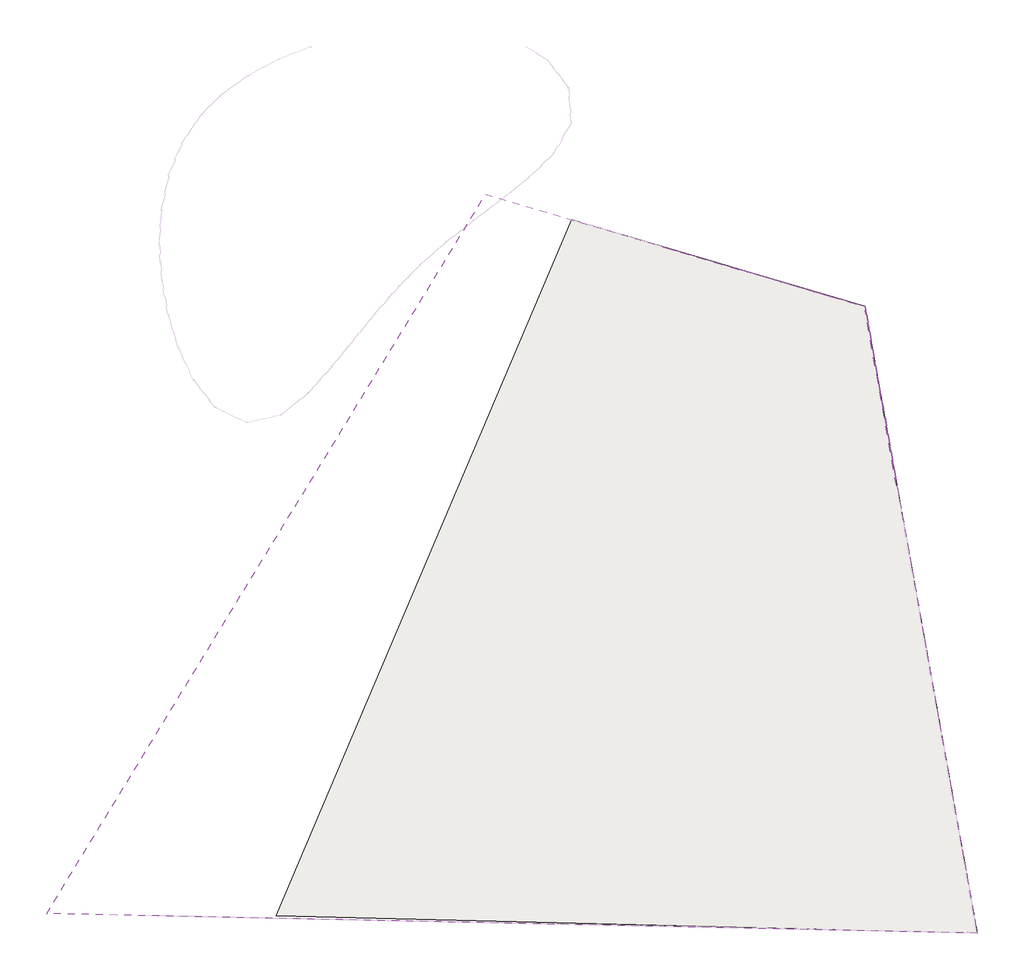
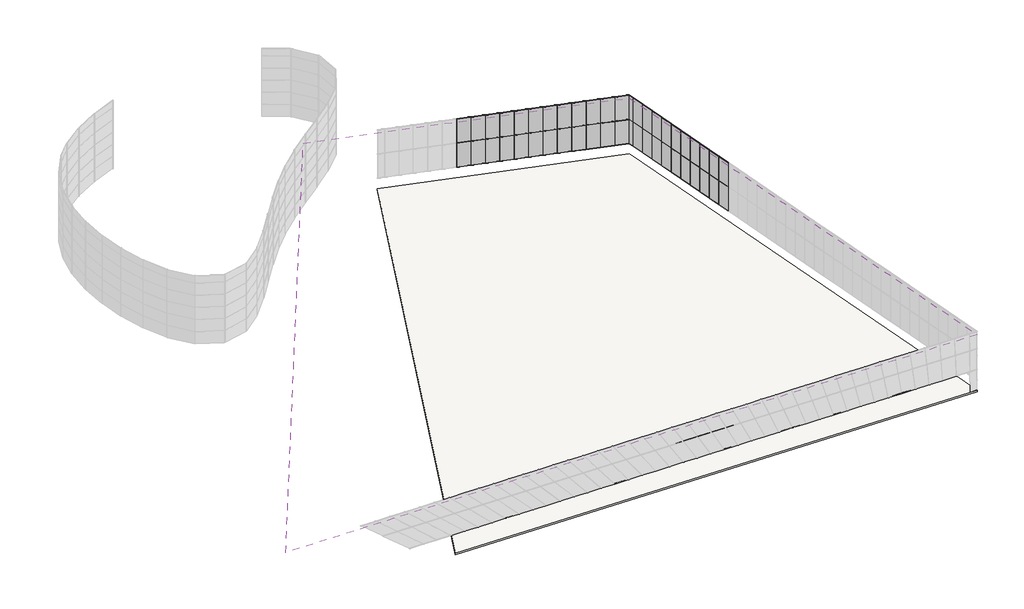
# One storey, part 8 of 8: 69 members, 46 plates, 1 roof, 1 slab.
"""IFC4 building model written with IfcOpenShell, lengths in millimetres."""

import ifcopenshell
import ifcopenshell.guid

model = None  # the IFC model being written
_history = None  # IfcOwnerHistory: only IFC2X3 demands one
_inside = {}  # id of a spatial element -> (the spatial element, [elements in it])
_under = {}  # id of a project, library or spatial element -> (it, [spatial elements below it])
_declared = {}  # id of a project -> (the project, [libraries it declares])
_typed = {}  # id of a type object -> (the type object, [elements of that type])
_made_of = {}  # id of a material, layer set ... -> (it, [elements and type objects made of it])


def new_model(schema):
    """Start an empty IFC model of exactly this schema.

    Asked for "IFC4X3", IfcOpenShell would pick the latest addendum, in which some entities
    have other attributes; the version numbers below select the first issue.
    IFC2X3 requires an IfcOwnerHistory on every rooted entity: one is made here for all.
    """
    global model, _history
    if schema == "IFC4X3":
        model = ifcopenshell.file(schema_version=(4, 3, 0, 0))
    else:
        model = ifcopenshell.file(schema=schema)
    _inside.clear()
    _under.clear()
    _declared.clear()
    _typed.clear()
    _made_of.clear()
    _history = None
    if model.schema == "IFC2X3":
        org = make("IfcOrganization", Name="unknown")
        user = make(
            "IfcPersonAndOrganization",
            ThePerson=make("IfcPerson", FamilyName="unknown"),
            TheOrganization=org,
        )
        app = make(
            "IfcApplication",
            ApplicationDeveloper=org,
            Version="unknown",
            ApplicationFullName="unknown",
            ApplicationIdentifier="unknown",
        )
        _history = make(
            "IfcOwnerHistory",
            OwningUser=user,
            OwningApplication=app,
            ChangeAction="ADDED",
            CreationDate=0,
        )
    return model


def make(cls, **values):
    """One entity of the class cls with the attributes given. An attribute that is None is left unset."""
    return model.create_entity(
        cls, **{name: value for name, value in values.items() if value is not None}
    )


def rooted(cls, **values):
    """An entity with a GlobalId (a new one), such as an element, a storey or a relation."""
    return make(cls, GlobalId=ifcopenshell.guid.new(), OwnerHistory=_history, **values)


def si_unit(unit_type, name, prefix=None):
    """IfcSIUnit, for example si_unit("LENGTHUNIT", "METRE", prefix="MILLI")."""
    return make("IfcSIUnit", UnitType=unit_type, Prefix=prefix, Name=name)


def assignment(units):
    """IfcUnitAssignment: the units of a project."""
    return None if units is None else make("IfcUnitAssignment", Units=units)


def point(xyz):
    """IfcCartesianPoint."""
    return None if xyz is None else make("IfcCartesianPoint", Coordinates=xyz)


def direction(xyz):
    """IfcDirection."""
    return None if xyz is None else make("IfcDirection", DirectionRatios=xyz)


def frame(location, z_axis=None, x_axis=None):
    """IfcAxis2Placement3D, a coordinate frame: its origin and axes. An axis left out is left unset."""
    return make(
        "IfcAxis2Placement3D",
        Location=point(location),
        Axis=direction(z_axis),
        RefDirection=direction(x_axis),
    )


def frame_2d(location, x_axis=None):
    """IfcAxis2Placement2D, a coordinate frame in the plane: its origin and x axis."""
    return make(
        "IfcAxis2Placement2D", Location=point(location), RefDirection=direction(x_axis)
    )


def origin():
    """The frame at (0, 0, 0) with its axes left unset."""
    return frame((0.0, 0.0, 0.0))


def origin_with_axes():
    """The frame at (0, 0, 0) with the z axis (0, 0, 1) and the x axis (1, 0, 0) written out."""
    return frame((0.0, 0.0, 0.0), z_axis=(0.0, 0.0, 1.0), x_axis=(1.0, 0.0, 0.0))


def origin_2d():
    """The frame at (0, 0) in the plane with its x axis left unset."""
    return frame_2d((0.0, 0.0))


def place(relative_to, where):
    """IfcLocalPlacement: puts the frame where relative to a parent placement (None: the world)."""
    return make(
        "IfcLocalPlacement", PlacementRelTo=relative_to, RelativePlacement=where
    )


def context(
    kind, dimensions, precision=None, world=None, true_north=None, identifier=None
):
    """IfcGeometricRepresentationContext, for example the 3D "Model" context."""
    return make(
        "IfcGeometricRepresentationContext",
        ContextIdentifier=identifier,
        ContextType=kind,
        CoordinateSpaceDimension=dimensions,
        Precision=precision,
        WorldCoordinateSystem=world,
        TrueNorth=true_north,
    )


def project(units=None, contexts=None):
    """IfcProject with its units and contexts."""
    return rooted(
        "IfcProject",
        Name="project",
        RepresentationContexts=contexts,
        UnitsInContext=assignment(units),
    )


def spatial(cls, under=None, at=None, **own):
    """A site, building, storey or space (cls), placed at a placement, below another one or the project."""
    s = rooted(cls, ObjectPlacement=at, **own)
    if under is not None:
        _under.setdefault(under.id(), (under, []))[1].append(s)
    return s


def polyline(points):
    """IfcPolyline through the points."""
    return make("IfcPolyline", Points=[point(p) for p in points])


def circle_curve(where, radius):
    """IfcCircle in the frame where."""
    return make("IfcCircle", Position=where, Radius=radius)


def trimmed(basis, trim1, trim2, sense, master):
    """IfcTrimmedCurve: the piece of a basis curve between two trims."""
    return make(
        "IfcTrimmedCurve",
        BasisCurve=basis,
        Trim1=trim1,
        Trim2=trim2,
        SenseAgreement=sense,
        MasterRepresentation=master,
    )


def segment(curve, same_sense, transition):
    """IfcCompositeCurveSegment."""
    return make(
        "IfcCompositeCurveSegment",
        Transition=transition,
        SameSense=same_sense,
        ParentCurve=curve,
    )


def composite_curve(segments, self_intersect=None):
    """IfcCompositeCurve: segments joined end to end."""
    return make("IfcCompositeCurve", Segments=segments, SelfIntersect=self_intersect)


def outline(outer, holes=None, kind="AREA"):
    """IfcArbitraryClosedProfileDef: a profile drawn as a closed curve; with holes, ...WithVoids."""
    if holes is None:
        return make("IfcArbitraryClosedProfileDef", ProfileType=kind, OuterCurve=outer)
    return make(
        "IfcArbitraryProfileDefWithVoids",
        ProfileType=kind,
        OuterCurve=outer,
        InnerCurves=holes,
    )


def extrude(swept, where, along, depth):
    """IfcExtrudedAreaSolid: the profile swept, set in the frame where, extruded along a direction by depth."""
    return make(
        "IfcExtrudedAreaSolid",
        SweptArea=swept,
        Position=where,
        ExtrudedDirection=direction(along),
        Depth=depth,
    )


def shape(context_of_items, identifier, shape_type, items):
    """IfcShapeRepresentation: the items that make up one representation, for example the "Body"."""
    return make(
        "IfcShapeRepresentation",
        ContextOfItems=context_of_items,
        RepresentationIdentifier=identifier,
        RepresentationType=shape_type,
        Items=items,
    )


def source(mapping_origin, context_of_items, identifier, shape_type, items):
    """IfcRepresentationMap: a shape defined once, which mapped items show again and again."""
    return make(
        "IfcRepresentationMap",
        MappingOrigin=mapping_origin,
        MappedRepresentation=shape(context_of_items, identifier, shape_type, items),
    )


def transform(
    local_origin,
    x_axis=None,
    y_axis=None,
    z_axis=None,
    scale=None,
    scale2=None,
    scale3=None,
    uniform=True,
):
    """IfcCartesianTransformationOperator3D, or its non-uniform kind. x_axis, y_axis, z_axis: its Axis1, 2, 3."""
    if uniform:
        return make(
            "IfcCartesianTransformationOperator3D",
            Axis1=direction(x_axis),
            Axis2=direction(y_axis),
            LocalOrigin=point(local_origin),
            Scale=scale,
            Axis3=direction(z_axis),
        )
    return make(
        "IfcCartesianTransformationOperator3DnonUniform",
        Axis1=direction(x_axis),
        Axis2=direction(y_axis),
        LocalOrigin=point(local_origin),
        Scale=scale,
        Axis3=direction(z_axis),
        Scale2=scale2,
        Scale3=scale3,
    )


def mapped(mapping_source, mapping_target):
    """IfcMappedItem: shows the shape of a source again, moved by a transform."""
    return make(
        "IfcMappedItem", MappingSource=mapping_source, MappingTarget=mapping_target
    )


def made_of(thing, what):
    """Note that an element or type object is made of a material, layer set ...; save() writes the relation."""
    if what is not None:
        _made_of.setdefault(what.id(), (what, []))[1].append(thing)
    return thing


def element(
    cls,
    number,
    at=None,
    inside=None,
    cuts=None,
    type_object=None,
    material=None,
    context=None,
    identifier="Body",
    shape_type=None,
    held_by="IfcProductDefinitionShape",
    body=None,
    shapes=None,
    **own,
):
    """One element of the class cls, such as IfcWall. Its Tag is "e" and its number.

    at: its placement. inside: the storey or other place that contains it. cuts: it is an
    opening in that element (IfcRelVoidsElement). A single representation is given by context,
    identifier, shape_type and body (its items); several are given by shapes. held_by: the class
    of the entity that holds the representations. save() writes the other relations.
    """
    e = rooted(cls, Tag="e%d" % number, ObjectPlacement=at, **own)
    if body is not None:
        shapes = [shape(context, identifier, shape_type, body)]
    if shapes is not None:
        e.Representation = make(held_by, Representations=shapes)
    if inside is not None:
        _inside.setdefault(inside.id(), (inside, []))[1].append(e)
    if cuts is not None:
        rooted(
            "IfcRelVoidsElement", RelatingBuildingElement=cuts, RelatedOpeningElement=e
        )
    if type_object is not None:
        _typed.setdefault(type_object.id(), (type_object, []))[1].append(e)
    return made_of(e, material)


def aggregate(whole, parts):
    """IfcRelAggregates: a whole, such as a stair, and the parts it consists of."""
    return rooted("IfcRelAggregates", RelatingObject=whole, RelatedObjects=parts)


def save(model, path):
    """Write the relations noted so far, then the file.

    IfcRelAggregates (storeys below a building ...), IfcRelContainedInSpatialStructure (elements
    in a storey), IfcRelDefinesByType, IfcRelAssociatesMaterial and IfcRelDeclares: one each for
    every whole, place, type object, material and project.
    """
    for whole, parts in _under.values():
        aggregate(whole, parts)
    for where, things in _inside.values():
        rooted(
            "IfcRelContainedInSpatialStructure",
            RelatedElements=things,
            RelatingStructure=where,
        )
    for kind, things in _typed.values():
        rooted("IfcRelDefinesByType", RelatedObjects=things, RelatingType=kind)
    for what, things in _made_of.values():
        rooted("IfcRelAssociatesMaterial", RelatedObjects=things, RelatingMaterial=what)
    for by, libraries in _declared.values():
        rooted("IfcRelDeclares", RelatingContext=by, RelatedDefinitions=libraries)
    model.write(path)


def montante_circular_25_mm_raio_666f7a7d(model_context):
    return source(origin(), model_context, "Body", "SweptSolid", [
        extrude(outline(composite_curve([segment(trimmed(circle_curve(frame_2d((-25.0, 0.0)), 25.0), [point((0.0, 0.0))], [point((-50.0, 0.0))], False, "CARTESIAN"), True, "CONTINUOUS"), segment(trimmed(circle_curve(frame_2d((-25.0, 0.0)), 25.0), [point((-50.0, 0.0))], [point((0.0, 0.0))], False, "CARTESIAN"), True, "CONTINUOUS")], self_intersect=False)), frame((0.0, 0.0, -685.7133319), z_axis=(0.0, 0.0, 1.0), x_axis=(1.0, 0.0, 0.0)), (0.0, 0.0, 1.0), 685.7133319),
    ])


def montante_circular_25_mm_raio_ce826986(model_context):
    return source(origin(), model_context, "Body", "SweptSolid", [
        extrude(outline(composite_curve([segment(trimmed(circle_curve(frame_2d((-25.0, 0.0)), 25.0), [point((0.0, 0.0))], [point((-50.0, 0.0))], False, "CARTESIAN"), True, "CONTINUOUS"), segment(trimmed(circle_curve(frame_2d((-25.0, 0.0)), 25.0), [point((-50.0, 0.0))], [point((0.0, 0.0))], False, "CARTESIAN"), True, "CONTINUOUS")], self_intersect=False)), frame((0.0, 0.0, -1500.0), z_axis=(0.0, 0.0, 1.0), x_axis=(1.0, 0.0, 0.0)), (0.0, 0.0, 1.0), 1500.0),
    ])


def montante_circular_25_mm_raio_36e581cf(model_context):
    return source(origin(), model_context, "Body", "SweptSolid", [
        extrude(outline(composite_curve([segment(trimmed(circle_curve(origin_2d(), 25.0), [point((25.0, 0.0))], [point((-25.0, 0.0))], False, "CARTESIAN"), True, "CONTINUOUS"), segment(trimmed(circle_curve(origin_2d(), 25.0), [point((-25.0, 0.0))], [point((25.0, 0.0))], False, "CARTESIAN"), True, "CONTINUOUS")], self_intersect=False)), frame((0.0, 0.0, -1500.0), z_axis=(0.0, 0.0, 1.0), x_axis=(1.0, 0.0, 0.0)), (0.0, 0.0, 1.0), 1500.0),
    ])


def montante_circular_25_mm_raio_b6a72e74(model_context):
    return source(origin(), model_context, "Body", "SweptSolid", [
        extrude(outline(composite_curve([segment(trimmed(circle_curve(origin_2d(), 25.0), [point((25.0, 0.0))], [point((-25.0, 0.0))], False, "CARTESIAN"), True, "CONTINUOUS"), segment(trimmed(circle_curve(origin_2d(), 25.0), [point((-25.0, 0.0))], [point((25.0, 0.0))], False, "CARTESIAN"), True, "CONTINUOUS")], self_intersect=False)), frame((0.0, 0.0, -685.7133319), z_axis=(0.0, 0.0, 1.0), x_axis=(1.0, 0.0, 0.0)), (0.0, 0.0, 1.0), 685.7133319),
    ])


def painel_do_sistema_5ef9eced(model_context):
    return source(origin(), model_context, "Body", "SweptSolid", [
        extrude(outline(polyline([(1475.0, 24.5), (-1475.0, 24.5), (-1475.0, 49.5), (1475.0, 49.5), (1475.0, 24.5)])), origin_with_axes(), (0.0, 0.0, 1.0), 1500.0),
    ])


def painel_do_sistema_14e00207(model_context):
    return source(origin(), model_context, "Body", "SweptSolid", [
        extrude(outline(polyline([(1475.0, 24.5), (-1475.0, 24.5), (-1475.0, 49.5), (1475.0, 49.5), (1475.0, 24.5)])), origin_with_axes(), (0.0, 0.0, 1.0), 685.7133319),
    ])


def painel_do_sistema_af596b93(model_context):
    return source(origin(), model_context, "Body", "SweptSolid", [
        extrude(outline(polyline([(1462.4999925, 24.5), (-1462.4999925, 24.5), (-1462.4999925, 49.5), (1462.4999925, 49.5), (1462.4999925, 24.5)])), origin_with_axes(), (0.0, 0.0, 1.0), 1500.0),
    ])


def painel_do_sistema_7f6e6910(model_context):
    return source(origin(), model_context, "Body", "SweptSolid", [
        extrude(outline(polyline([(1462.4999925, 24.5), (-1462.4999925, 24.5), (-1462.4999925, 49.5), (1462.4999925, 49.5), (1462.4999925, 24.5)])), origin_with_axes(), (0.0, 0.0, 1.0), 685.7133319),
    ])


model = new_model("IFC4")

# Units and contexts
model_context = context("Model", 3, world=origin())
ifc_project = project(units=[si_unit("LENGTHUNIT", "METRE", prefix="MILLI")], contexts=[model_context])

# Site, building, storey
site = spatial("IfcSite", under=ifc_project)
building = spatial("IfcBuilding", under=site)
storey = spatial("IfcBuildingStorey", under=building, Name="Nível 3", Elevation=7695.2)

# Members
placement = place(None, origin())
montante_circular_25_mm_raio_shape = montante_circular_25_mm_raio_666f7a7d(model_context)
element("IfcMember", 1, ObjectType="Montante circular : 25 mm Raio", at=placement, inside=storey, context=model_context, shape_type="MappedRepresentation", body=[
    mapped(montante_circular_25_mm_raio_shape, transform((18627.8077271, 25569.7371494, 15000.0), x_axis=(0.0, 0.0, 1.0), y_axis=(0.9843520034862613, 0.17621331740984683, 0.0), z_axis=(-0.17621331740984683, 0.9843520034862613, 0.0))),
])
montante_circular_25_mm_raio_2_shape = montante_circular_25_mm_raio_ce826986(model_context)
element("IfcMember", 2, ObjectType="Montante circular : 25 mm Raio", at=placement, inside=storey, context=model_context, shape_type="MappedRepresentation", body=[
    mapped(montante_circular_25_mm_raio_2_shape, transform((17189.2092362, 25994.5128335, 15000.0), x_axis=(0.0, 0.0, 1.0), y_axis=(0.2831837893953463, 0.9590656606425298, 0.0), z_axis=(-0.9590656606425297, 0.2831837893953462, 0.0))),
])
element("IfcMember", 3, ObjectType="Montante circular : 25 mm Raio", at=placement, inside=storey, context=model_context, shape_type="MappedRepresentation", body=[
    mapped(montante_circular_25_mm_raio_2_shape, transform((21127.5193332, 11606.0018103, 15000.0), x_axis=(0.0, 0.0, 1.0), y_axis=(0.9843520034862614, 0.17621331740984636, 0.0), z_axis=(-0.17621331740984636, 0.9843520034862614, 0.0))),
])
element("IfcMember", 4, ObjectType="Montante circular : 25 mm Raio", at=placement, inside=storey, context=model_context, shape_type="MappedRepresentation", body=[
    mapped(montante_circular_25_mm_raio_2_shape, transform((20863.1993571, 13082.5298156, 15000.0), x_axis=(0.0, 0.0, 1.0), y_axis=(0.9843520034862611, 0.17621331740984836, 0.0), z_axis=(-0.17621331740984836, 0.9843520034862611, 0.0))),
])
element("IfcMember", 5, ObjectType="Montante circular : 25 mm Raio", at=placement, inside=storey, context=model_context, shape_type="MappedRepresentation", body=[
    mapped(montante_circular_25_mm_raio_2_shape, transform((20598.8793809, 14559.0578208, 15000.0), x_axis=(0.0, 0.0, 1.0), y_axis=(0.9843520034862613, 0.17621331740984736, 0.0), z_axis=(-0.17621331740984733, 0.9843520034862612, 0.0))),
])
element("IfcMember", 6, ObjectType="Montante circular : 25 mm Raio", at=placement, inside=storey, context=model_context, shape_type="MappedRepresentation", body=[
    mapped(montante_circular_25_mm_raio_2_shape, transform((20334.5594048, 16035.585826, 15000.0), x_axis=(0.0, 0.0, 1.0), y_axis=(0.9843520034862608, 0.17621331740984966, 0.0), z_axis=(-0.17621331740984966, 0.9843520034862608, 0.0))),
])
element("IfcMember", 7, ObjectType="Montante circular : 25 mm Raio", at=placement, inside=storey, context=model_context, shape_type="MappedRepresentation", body=[
    mapped(montante_circular_25_mm_raio_2_shape, transform((20070.2394287, 17512.1138312, 15000.0), x_axis=(0.0, 0.0, 1.0), y_axis=(0.9843520034862613, 0.1762133174098471, 0.0), z_axis=(-0.17621331740984708, 0.9843520034862612, 0.0))),
])
element("IfcMember", 8, ObjectType="Montante circular : 25 mm Raio", at=placement, inside=storey, context=model_context, shape_type="MappedRepresentation", body=[
    mapped(montante_circular_25_mm_raio_2_shape, transform((19805.9194526, 18988.6418365, 15000.0), x_axis=(0.0, 0.0, 1.0), y_axis=(0.9843520034862611, 0.17621331740984836, 0.0), z_axis=(-0.17621331740984836, 0.9843520034862611, 0.0))),
])
element("IfcMember", 9, ObjectType="Montante circular : 25 mm Raio", at=placement, inside=storey, context=model_context, shape_type="MappedRepresentation", body=[
    mapped(montante_circular_25_mm_raio_2_shape, transform((19541.5994765, 20465.1698417, 15000.0), x_axis=(0.0, 0.0, 1.0), y_axis=(0.9843520034862608, 0.1762133174098494, 0.0), z_axis=(-0.1762133174098494, 0.9843520034862608, 0.0))),
])
element("IfcMember", 10, ObjectType="Montante circular : 25 mm Raio", at=placement, inside=storey, context=model_context, shape_type="MappedRepresentation", body=[
    mapped(montante_circular_25_mm_raio_2_shape, transform((19277.2795004, 21941.6978469, 15000.0), x_axis=(0.0, 0.0, 1.0), y_axis=(0.9843520034862612, 0.1762133174098476, 0.0), z_axis=(-0.1762133174098476, 0.9843520034862612, 0.0))),
])
element("IfcMember", 11, ObjectType="Montante circular : 25 mm Raio", at=placement, inside=storey, context=model_context, shape_type="MappedRepresentation", body=[
    mapped(montante_circular_25_mm_raio_2_shape, transform((19012.9595243, 23418.2258522, 15000.0), x_axis=(0.0, 0.0, 1.0), y_axis=(0.9843520034862611, 0.1762133174098481, 0.0), z_axis=(-0.1762133174098481, 0.9843520034862611, 0.0))),
])
element("IfcMember", 12, ObjectType="Montante circular : 25 mm Raio", at=placement, inside=storey, context=model_context, shape_type="MappedRepresentation", body=[
    mapped(montante_circular_25_mm_raio_2_shape, transform((18748.6395481, 24894.7538574, 15000.0), x_axis=(0.0, 0.0, 1.0), y_axis=(0.9843520034862611, 0.1762133174098484, 0.0), z_axis=(-0.17621331740984839, 0.984352003486261, 0.0))),
])
element("IfcMember", 13, ObjectType="Montante circular : 25 mm Raio", at=placement, inside=storey, context=model_context, shape_type="MappedRepresentation", body=[
    mapped(montante_circular_25_mm_raio_2_shape, transform((15750.6107452, 26419.2885176, 15000.0), x_axis=(0.0, 0.0, 1.0), y_axis=(0.28318378939534644, 0.9590656606425298, 0.0), z_axis=(-0.9590656606425298, 0.28318378939534644, 0.0))),
])
element("IfcMember", 14, ObjectType="Montante circular : 25 mm Raio", at=placement, inside=storey, context=model_context, shape_type="MappedRepresentation", body=[
    mapped(montante_circular_25_mm_raio_2_shape, transform((14312.0122543, 26844.0642017, 15000.0), x_axis=(0.0, 0.0, 1.0), y_axis=(0.2831837893953491, 0.959065660642529, 0.0), z_axis=(-0.959065660642529, 0.2831837893953491, 0.0))),
])
element("IfcMember", 15, ObjectType="Montante circular : 25 mm Raio", at=placement, inside=storey, context=model_context, shape_type="MappedRepresentation", body=[
    mapped(montante_circular_25_mm_raio_2_shape, transform((12873.4137633, 27268.8398858, 15000.0), x_axis=(0.0, 0.0, 1.0), y_axis=(0.2831837893953487, 0.9590656606425292, 0.0), z_axis=(-0.9590656606425291, 0.28318378939534866, 0.0))),
])
element("IfcMember", 16, ObjectType="Montante circular : 25 mm Raio", at=placement, inside=storey, context=model_context, shape_type="MappedRepresentation", body=[
    mapped(montante_circular_25_mm_raio_2_shape, transform((11434.8152723, 27693.6155699, 15000.0), x_axis=(0.0, 0.0, 1.0), y_axis=(0.2831837893953472, 0.9590656606425295, 0.0), z_axis=(-0.9590656606425295, 0.2831837893953472, 0.0))),
])
element("IfcMember", 17, ObjectType="Montante circular : 25 mm Raio", at=placement, inside=storey, context=model_context, shape_type="MappedRepresentation", body=[
    mapped(montante_circular_25_mm_raio_2_shape, transform((9996.2167814, 28118.391254, 15000.0), x_axis=(0.0, 0.0, 1.0), y_axis=(0.2831837893953487, 0.9590656606425292, 0.0), z_axis=(-0.9590656606425291, 0.28318378939534866, 0.0))),
])
element("IfcMember", 18, ObjectType="Montante circular : 25 mm Raio", at=placement, inside=storey, context=model_context, shape_type="MappedRepresentation", body=[
    mapped(montante_circular_25_mm_raio_2_shape, transform((8557.6182904, 28543.1669381, 15000.0), x_axis=(0.0, 0.0, 1.0), y_axis=(0.28318378939534666, 0.9590656606425297, 0.0), z_axis=(-0.9590656606425296, 0.2831837893953466, 0.0))),
])
element("IfcMember", 19, ObjectType="Montante circular : 25 mm Raio", at=placement, inside=storey, context=model_context, shape_type="MappedRepresentation", body=[
    mapped(montante_circular_25_mm_raio_2_shape, transform((7119.0197994, 28967.9426222, 15000.0), x_axis=(0.0, 0.0, 1.0), y_axis=(0.2831837893953493, 0.959065660642529, 0.0), z_axis=(-0.959065660642529, 0.2831837893953493, 0.0))),
])
element("IfcMember", 20, ObjectType="Montante circular : 25 mm Raio", at=placement, inside=storey, context=model_context, shape_type="MappedRepresentation", body=[
    mapped(montante_circular_25_mm_raio_2_shape, transform((5680.4213085, 29392.7183063, 15000.0), x_axis=(0.0, 0.0, 1.0), y_axis=(0.2831837893953491, 0.959065660642529, 0.0), z_axis=(-0.959065660642529, 0.2831837893953491, 0.0))),
])
element("IfcMember", 21, ObjectType="Montante circular : 25 mm Raio", at=placement, inside=storey, context=model_context, shape_type="MappedRepresentation", body=[
    mapped(montante_circular_25_mm_raio_2_shape, transform((4241.8228175, 29817.4939904, 15000.0), x_axis=(0.0, 0.0, 1.0), y_axis=(0.28318378939534394, 0.9590656606425305, 0.0), z_axis=(-0.9590656606425305, 0.28318378939534394, 0.0))),
])
element("IfcMember", 22, ObjectType="Montante circular : 25 mm Raio", at=placement, inside=storey, context=model_context, shape_type="MappedRepresentation", body=[
    mapped(montante_circular_25_mm_raio_2_shape, transform((2803.2243265, 30242.2696745, 15000.0), x_axis=(0.0, 0.0, 1.0), y_axis=(0.28318378939535055, 0.9590656606425285, 0.0), z_axis=(-0.9590656606425285, 0.28318378939535055, 0.0))),
])
element("IfcMember", 23, ObjectType="Montante circular : 25 mm Raio", at=placement, inside=storey, context=model_context, shape_type="MappedRepresentation", body=[
    mapped(montante_circular_25_mm_raio_2_shape, transform((1364.6258356, 30667.0453586, 15000.0), x_axis=(0.0, 0.0, 1.0), y_axis=(0.28318378939534655, 0.9590656606425297, 0.0), z_axis=(-0.9590656606425296, 0.2831837893953465, 0.0))),
])
montante_circular_25_mm_raio_3_shape = montante_circular_25_mm_raio_36e581cf(model_context)
element("IfcMember", 24, ObjectType="Montante circular : 25 mm Raio", at=placement, inside=storey, context=model_context, shape_type="MappedRepresentation", body=[
    mapped(montante_circular_25_mm_raio_3_shape, transform((17189.2092362, 25994.5128335, 9000.000015), x_axis=(0.0, 0.0, 1.0), y_axis=(0.2831837893953463, 0.9590656606425298, 0.0), z_axis=(-0.9590656606425297, 0.2831837893953462, 0.0))),
])
element("IfcMember", 25, ObjectType="Montante circular : 25 mm Raio", at=placement, inside=storey, context=model_context, shape_type="MappedRepresentation", body=[
    mapped(montante_circular_25_mm_raio_3_shape, transform((17189.2092362, 25994.5128335, 12000.000015), x_axis=(0.0, 0.0, 1.0), y_axis=(0.2831837893953463, 0.9590656606425298, 0.0), z_axis=(-0.9590656606425297, 0.2831837893953462, 0.0))),
])
element("IfcMember", 26, ObjectType="Montante circular : 25 mm Raio", at=placement, inside=storey, context=model_context, shape_type="MappedRepresentation", body=[
    mapped(montante_circular_25_mm_raio_3_shape, transform((21127.5193332, 11606.0018103, 9000.000015), x_axis=(0.0, 0.0, 1.0), y_axis=(0.9843520034862615, 0.17621331740984614, 0.0), z_axis=(-0.1762133174098461, 0.9843520034862614, 0.0))),
])
element("IfcMember", 27, ObjectType="Montante circular : 25 mm Raio", at=placement, inside=storey, context=model_context, shape_type="MappedRepresentation", body=[
    mapped(montante_circular_25_mm_raio_3_shape, transform((20863.1993571, 13082.5298156, 9000.000015), x_axis=(0.0, 0.0, 1.0), y_axis=(0.9843520034862611, 0.1762133174098486, 0.0), z_axis=(-0.1762133174098486, 0.9843520034862611, 0.0))),
])
element("IfcMember", 28, ObjectType="Montante circular : 25 mm Raio", at=placement, inside=storey, context=model_context, shape_type="MappedRepresentation", body=[
    mapped(montante_circular_25_mm_raio_3_shape, transform((20598.8793809, 14559.0578208, 9000.000015), x_axis=(0.0, 0.0, 1.0), y_axis=(0.9843520034862613, 0.17621331740984736, 0.0), z_axis=(-0.17621331740984733, 0.9843520034862612, 0.0))),
])
element("IfcMember", 29, ObjectType="Montante circular : 25 mm Raio", at=placement, inside=storey, context=model_context, shape_type="MappedRepresentation", body=[
    mapped(montante_circular_25_mm_raio_3_shape, transform((20334.5594048, 16035.585826, 9000.000015), x_axis=(0.0, 0.0, 1.0), y_axis=(0.9843520034862608, 0.17621331740984966, 0.0), z_axis=(-0.17621331740984966, 0.9843520034862608, 0.0))),
])
element("IfcMember", 30, ObjectType="Montante circular : 25 mm Raio", at=placement, inside=storey, context=model_context, shape_type="MappedRepresentation", body=[
    mapped(montante_circular_25_mm_raio_3_shape, transform((20070.2394287, 17512.1138312, 9000.000015), x_axis=(0.0, 0.0, 1.0), y_axis=(0.9843520034862613, 0.1762133174098471, 0.0), z_axis=(-0.17621331740984708, 0.9843520034862612, 0.0))),
])
element("IfcMember", 31, ObjectType="Montante circular : 25 mm Raio", at=placement, inside=storey, context=model_context, shape_type="MappedRepresentation", body=[
    mapped(montante_circular_25_mm_raio_3_shape, transform((19805.9194526, 18988.6418365, 9000.000015), x_axis=(0.0, 0.0, 1.0), y_axis=(0.9843520034862611, 0.17621331740984836, 0.0), z_axis=(-0.17621331740984836, 0.9843520034862611, 0.0))),
])
element("IfcMember", 32, ObjectType="Montante circular : 25 mm Raio", at=placement, inside=storey, context=model_context, shape_type="MappedRepresentation", body=[
    mapped(montante_circular_25_mm_raio_3_shape, transform((19541.5994765, 20465.1698417, 9000.000015), x_axis=(0.0, 0.0, 1.0), y_axis=(0.9843520034862608, 0.1762133174098494, 0.0), z_axis=(-0.1762133174098494, 0.9843520034862608, 0.0))),
])
element("IfcMember", 33, ObjectType="Montante circular : 25 mm Raio", at=placement, inside=storey, context=model_context, shape_type="MappedRepresentation", body=[
    mapped(montante_circular_25_mm_raio_3_shape, transform((19277.2795004, 21941.6978469, 9000.000015), x_axis=(0.0, 0.0, 1.0), y_axis=(0.9843520034862612, 0.1762133174098476, 0.0), z_axis=(-0.1762133174098476, 0.9843520034862612, 0.0))),
])
element("IfcMember", 34, ObjectType="Montante circular : 25 mm Raio", at=placement, inside=storey, context=model_context, shape_type="MappedRepresentation", body=[
    mapped(montante_circular_25_mm_raio_3_shape, transform((19012.9595243, 23418.2258522, 9000.000015), x_axis=(0.0, 0.0, 1.0), y_axis=(0.9843520034862611, 0.1762133174098481, 0.0), z_axis=(-0.1762133174098481, 0.9843520034862611, 0.0))),
])
element("IfcMember", 35, ObjectType="Montante circular : 25 mm Raio", at=placement, inside=storey, context=model_context, shape_type="MappedRepresentation", body=[
    mapped(montante_circular_25_mm_raio_3_shape, transform((18748.6395481, 24894.7538574, 9000.000015), x_axis=(0.0, 0.0, 1.0), y_axis=(0.9843520034862611, 0.1762133174098484, 0.0), z_axis=(-0.17621331740984839, 0.984352003486261, 0.0))),
])
element("IfcMember", 36, ObjectType="Montante circular : 25 mm Raio", at=placement, inside=storey, context=model_context, shape_type="MappedRepresentation", body=[
    mapped(montante_circular_25_mm_raio_3_shape, transform((21127.5193332, 11606.0018103, 12000.000015), x_axis=(0.0, 0.0, 1.0), y_axis=(0.9843520034862615, 0.17621331740984614, 0.0), z_axis=(-0.1762133174098461, 0.9843520034862614, 0.0))),
])
element("IfcMember", 37, ObjectType="Montante circular : 25 mm Raio", at=placement, inside=storey, context=model_context, shape_type="MappedRepresentation", body=[
    mapped(montante_circular_25_mm_raio_3_shape, transform((20863.1993571, 13082.5298156, 12000.000015), x_axis=(0.0, 0.0, 1.0), y_axis=(0.9843520034862611, 0.1762133174098486, 0.0), z_axis=(-0.1762133174098486, 0.9843520034862611, 0.0))),
])
element("IfcMember", 38, ObjectType="Montante circular : 25 mm Raio", at=placement, inside=storey, context=model_context, shape_type="MappedRepresentation", body=[
    mapped(montante_circular_25_mm_raio_3_shape, transform((20598.8793809, 14559.0578208, 12000.000015), x_axis=(0.0, 0.0, 1.0), y_axis=(0.9843520034862613, 0.17621331740984736, 0.0), z_axis=(-0.17621331740984733, 0.9843520034862612, 0.0))),
])
element("IfcMember", 39, ObjectType="Montante circular : 25 mm Raio", at=placement, inside=storey, context=model_context, shape_type="MappedRepresentation", body=[
    mapped(montante_circular_25_mm_raio_3_shape, transform((20334.5594048, 16035.585826, 12000.000015), x_axis=(0.0, 0.0, 1.0), y_axis=(0.9843520034862608, 0.17621331740984966, 0.0), z_axis=(-0.17621331740984966, 0.9843520034862608, 0.0))),
])
element("IfcMember", 40, ObjectType="Montante circular : 25 mm Raio", at=placement, inside=storey, context=model_context, shape_type="MappedRepresentation", body=[
    mapped(montante_circular_25_mm_raio_3_shape, transform((20070.2394287, 17512.1138312, 12000.000015), x_axis=(0.0, 0.0, 1.0), y_axis=(0.9843520034862613, 0.1762133174098471, 0.0), z_axis=(-0.17621331740984708, 0.9843520034862612, 0.0))),
])
element("IfcMember", 41, ObjectType="Montante circular : 25 mm Raio", at=placement, inside=storey, context=model_context, shape_type="MappedRepresentation", body=[
    mapped(montante_circular_25_mm_raio_3_shape, transform((19805.9194526, 18988.6418365, 12000.000015), x_axis=(0.0, 0.0, 1.0), y_axis=(0.9843520034862611, 0.17621331740984836, 0.0), z_axis=(-0.17621331740984836, 0.9843520034862611, 0.0))),
])
element("IfcMember", 42, ObjectType="Montante circular : 25 mm Raio", at=placement, inside=storey, context=model_context, shape_type="MappedRepresentation", body=[
    mapped(montante_circular_25_mm_raio_3_shape, transform((19541.5994765, 20465.1698417, 12000.000015), x_axis=(0.0, 0.0, 1.0), y_axis=(0.9843520034862608, 0.1762133174098494, 0.0), z_axis=(-0.1762133174098494, 0.9843520034862608, 0.0))),
])
element("IfcMember", 43, ObjectType="Montante circular : 25 mm Raio", at=placement, inside=storey, context=model_context, shape_type="MappedRepresentation", body=[
    mapped(montante_circular_25_mm_raio_3_shape, transform((19277.2795004, 21941.6978469, 12000.000015), x_axis=(0.0, 0.0, 1.0), y_axis=(0.9843520034862612, 0.1762133174098476, 0.0), z_axis=(-0.1762133174098476, 0.9843520034862612, 0.0))),
])
element("IfcMember", 44, ObjectType="Montante circular : 25 mm Raio", at=placement, inside=storey, context=model_context, shape_type="MappedRepresentation", body=[
    mapped(montante_circular_25_mm_raio_3_shape, transform((19012.9595243, 23418.2258522, 12000.000015), x_axis=(0.0, 0.0, 1.0), y_axis=(0.9843520034862611, 0.1762133174098481, 0.0), z_axis=(-0.1762133174098481, 0.9843520034862611, 0.0))),
])
element("IfcMember", 45, ObjectType="Montante circular : 25 mm Raio", at=placement, inside=storey, context=model_context, shape_type="MappedRepresentation", body=[
    mapped(montante_circular_25_mm_raio_3_shape, transform((18748.6395481, 24894.7538574, 12000.000015), x_axis=(0.0, 0.0, 1.0), y_axis=(0.9843520034862611, 0.1762133174098484, 0.0), z_axis=(-0.17621331740984839, 0.984352003486261, 0.0))),
])
element("IfcMember", 46, ObjectType="Montante circular : 25 mm Raio", at=placement, inside=storey, context=model_context, shape_type="MappedRepresentation", body=[
    mapped(montante_circular_25_mm_raio_3_shape, transform((15750.6107452, 26419.2885176, 9000.000015), x_axis=(0.0, 0.0, 1.0), y_axis=(0.28318378939534644, 0.9590656606425298, 0.0), z_axis=(-0.9590656606425298, 0.28318378939534644, 0.0))),
])
element("IfcMember", 47, ObjectType="Montante circular : 25 mm Raio", at=placement, inside=storey, context=model_context, shape_type="MappedRepresentation", body=[
    mapped(montante_circular_25_mm_raio_3_shape, transform((14312.0122543, 26844.0642017, 9000.000015), x_axis=(0.0, 0.0, 1.0), y_axis=(0.2831837893953491, 0.959065660642529, 0.0), z_axis=(-0.959065660642529, 0.2831837893953491, 0.0))),
])
element("IfcMember", 48, ObjectType="Montante circular : 25 mm Raio", at=placement, inside=storey, context=model_context, shape_type="MappedRepresentation", body=[
    mapped(montante_circular_25_mm_raio_3_shape, transform((12873.4137633, 27268.8398858, 9000.000015), x_axis=(0.0, 0.0, 1.0), y_axis=(0.2831837893953487, 0.9590656606425292, 0.0), z_axis=(-0.9590656606425291, 0.28318378939534866, 0.0))),
])
element("IfcMember", 49, ObjectType="Montante circular : 25 mm Raio", at=placement, inside=storey, context=model_context, shape_type="MappedRepresentation", body=[
    mapped(montante_circular_25_mm_raio_3_shape, transform((11434.8152723, 27693.6155699, 9000.000015), x_axis=(0.0, 0.0, 1.0), y_axis=(0.2831837893953472, 0.9590656606425295, 0.0), z_axis=(-0.9590656606425295, 0.2831837893953472, 0.0))),
])
element("IfcMember", 50, ObjectType="Montante circular : 25 mm Raio", at=placement, inside=storey, context=model_context, shape_type="MappedRepresentation", body=[
    mapped(montante_circular_25_mm_raio_3_shape, transform((9996.2167814, 28118.391254, 9000.000015), x_axis=(0.0, 0.0, 1.0), y_axis=(0.2831837893953487, 0.9590656606425292, 0.0), z_axis=(-0.9590656606425291, 0.28318378939534866, 0.0))),
])
element("IfcMember", 51, ObjectType="Montante circular : 25 mm Raio", at=placement, inside=storey, context=model_context, shape_type="MappedRepresentation", body=[
    mapped(montante_circular_25_mm_raio_3_shape, transform((8557.6182904, 28543.1669381, 9000.000015), x_axis=(0.0, 0.0, 1.0), y_axis=(0.28318378939534666, 0.9590656606425297, 0.0), z_axis=(-0.9590656606425296, 0.2831837893953466, 0.0))),
])
element("IfcMember", 52, ObjectType="Montante circular : 25 mm Raio", at=placement, inside=storey, context=model_context, shape_type="MappedRepresentation", body=[
    mapped(montante_circular_25_mm_raio_3_shape, transform((7119.0197994, 28967.9426222, 9000.000015), x_axis=(0.0, 0.0, 1.0), y_axis=(0.2831837893953493, 0.959065660642529, 0.0), z_axis=(-0.959065660642529, 0.2831837893953493, 0.0))),
])
element("IfcMember", 53, ObjectType="Montante circular : 25 mm Raio", at=placement, inside=storey, context=model_context, shape_type="MappedRepresentation", body=[
    mapped(montante_circular_25_mm_raio_3_shape, transform((5680.4213085, 29392.7183063, 9000.000015), x_axis=(0.0, 0.0, 1.0), y_axis=(0.2831837893953491, 0.959065660642529, 0.0), z_axis=(-0.959065660642529, 0.2831837893953491, 0.0))),
])
element("IfcMember", 54, ObjectType="Montante circular : 25 mm Raio", at=placement, inside=storey, context=model_context, shape_type="MappedRepresentation", body=[
    mapped(montante_circular_25_mm_raio_3_shape, transform((4241.8228175, 29817.4939904, 9000.000015), x_axis=(0.0, 0.0, 1.0), y_axis=(0.28318378939534394, 0.9590656606425305, 0.0), z_axis=(-0.9590656606425305, 0.28318378939534394, 0.0))),
])
element("IfcMember", 55, ObjectType="Montante circular : 25 mm Raio", at=placement, inside=storey, context=model_context, shape_type="MappedRepresentation", body=[
    mapped(montante_circular_25_mm_raio_3_shape, transform((2803.2243265, 30242.2696745, 9000.000015), x_axis=(0.0, 0.0, 1.0), y_axis=(0.28318378939535077, 0.9590656606425285, 0.0), z_axis=(-0.9590656606425284, 0.2831837893953507, 0.0))),
])
element("IfcMember", 56, ObjectType="Montante circular : 25 mm Raio", at=placement, inside=storey, context=model_context, shape_type="MappedRepresentation", body=[
    mapped(montante_circular_25_mm_raio_3_shape, transform((1364.6258356, 30667.0453586, 9000.000015), x_axis=(0.0, 0.0, 1.0), y_axis=(0.28318378939534655, 0.9590656606425297, 0.0), z_axis=(-0.9590656606425296, 0.2831837893953465, 0.0))),
])
element("IfcMember", 57, ObjectType="Montante circular : 25 mm Raio", at=placement, inside=storey, context=model_context, shape_type="MappedRepresentation", body=[
    mapped(montante_circular_25_mm_raio_3_shape, transform((15750.6107452, 26419.2885176, 12000.000015), x_axis=(0.0, 0.0, 1.0), y_axis=(0.2831837893953491, 0.959065660642529, 0.0), z_axis=(-0.959065660642529, 0.2831837893953491, 0.0))),
])
element("IfcMember", 58, ObjectType="Montante circular : 25 mm Raio", at=placement, inside=storey, context=model_context, shape_type="MappedRepresentation", body=[
    mapped(montante_circular_25_mm_raio_3_shape, transform((14312.0122543, 26844.0642017, 12000.000015), x_axis=(0.0, 0.0, 1.0), y_axis=(0.28318378939534383, 0.9590656606425306, 0.0), z_axis=(-0.9590656606425305, 0.2831837893953438, 0.0))),
])
element("IfcMember", 59, ObjectType="Montante circular : 25 mm Raio", at=placement, inside=storey, context=model_context, shape_type="MappedRepresentation", body=[
    mapped(montante_circular_25_mm_raio_3_shape, transform((12873.4137633, 27268.8398858, 12000.000015), x_axis=(0.0, 0.0, 1.0), y_axis=(0.2831837893953487, 0.9590656606425292, 0.0), z_axis=(-0.9590656606425291, 0.28318378939534866, 0.0))),
])
element("IfcMember", 60, ObjectType="Montante circular : 25 mm Raio", at=placement, inside=storey, context=model_context, shape_type="MappedRepresentation", body=[
    mapped(montante_circular_25_mm_raio_3_shape, transform((11434.8152723, 27693.6155699, 12000.000015), x_axis=(0.0, 0.0, 1.0), y_axis=(0.2831837893953498, 0.9590656606425287, 0.0), z_axis=(-0.9590656606425287, 0.2831837893953498, 0.0))),
])
element("IfcMember", 61, ObjectType="Montante circular : 25 mm Raio", at=placement, inside=storey, context=model_context, shape_type="MappedRepresentation", body=[
    mapped(montante_circular_25_mm_raio_3_shape, transform((9996.2167814, 28118.391254, 12000.000015), x_axis=(0.0, 0.0, 1.0), y_axis=(0.2831837893953487, 0.9590656606425292, 0.0), z_axis=(-0.9590656606425291, 0.28318378939534866, 0.0))),
])
element("IfcMember", 62, ObjectType="Montante circular : 25 mm Raio", at=placement, inside=storey, context=model_context, shape_type="MappedRepresentation", body=[
    mapped(montante_circular_25_mm_raio_3_shape, transform((8557.6182904, 28543.1669381, 12000.000015), x_axis=(0.0, 0.0, 1.0), y_axis=(0.28318378939534666, 0.9590656606425297, 0.0), z_axis=(-0.9590656606425296, 0.2831837893953466, 0.0))),
])
element("IfcMember", 63, ObjectType="Montante circular : 25 mm Raio", at=placement, inside=storey, context=model_context, shape_type="MappedRepresentation", body=[
    mapped(montante_circular_25_mm_raio_3_shape, transform((7119.0197994, 28967.9426222, 12000.000015), x_axis=(0.0, 0.0, 1.0), y_axis=(0.28318378939535177, 0.9590656606425283, 0.0), z_axis=(-0.9590656606425283, 0.28318378939535177, 0.0))),
])
element("IfcMember", 64, ObjectType="Montante circular : 25 mm Raio", at=placement, inside=storey, context=model_context, shape_type="MappedRepresentation", body=[
    mapped(montante_circular_25_mm_raio_3_shape, transform((5680.4213085, 29392.7183063, 12000.000015), x_axis=(0.0, 0.0, 1.0), y_axis=(0.28318378939534644, 0.9590656606425298, 0.0), z_axis=(-0.9590656606425298, 0.28318378939534644, 0.0))),
])
element("IfcMember", 65, ObjectType="Montante circular : 25 mm Raio", at=placement, inside=storey, context=model_context, shape_type="MappedRepresentation", body=[
    mapped(montante_circular_25_mm_raio_3_shape, transform((4241.8228175, 29817.4939904, 12000.000015), x_axis=(0.0, 0.0, 1.0), y_axis=(0.28318378939534655, 0.9590656606425297, 0.0), z_axis=(-0.9590656606425296, 0.2831837893953465, 0.0))),
])
element("IfcMember", 66, ObjectType="Montante circular : 25 mm Raio", at=placement, inside=storey, context=model_context, shape_type="MappedRepresentation", body=[
    mapped(montante_circular_25_mm_raio_3_shape, transform((2803.2243265, 30242.2696745, 12000.000015), x_axis=(0.0, 0.0, 1.0), y_axis=(0.28318378939535077, 0.9590656606425285, 0.0), z_axis=(-0.9590656606425284, 0.2831837893953507, 0.0))),
])
element("IfcMember", 67, ObjectType="Montante circular : 25 mm Raio", at=placement, inside=storey, context=model_context, shape_type="MappedRepresentation", body=[
    mapped(montante_circular_25_mm_raio_3_shape, transform((1364.6258356, 30667.0453586, 12000.000015), x_axis=(0.0, 0.0, 1.0), y_axis=(0.2831837893953466, 0.9590656606425297, 0.0), z_axis=(-0.9590656606425296, 0.28318378939534655, 0.0))),
])
montante_circular_25_mm_raio_4_shape = montante_circular_25_mm_raio_b6a72e74(model_context)
element("IfcMember", 68, ObjectType="Montante circular : 25 mm Raio", at=placement, inside=storey, context=model_context, shape_type="MappedRepresentation", body=[
    mapped(montante_circular_25_mm_raio_4_shape, transform((18627.8077271, 25569.7371494, 9000.000015), x_axis=(0.0, 0.0, 1.0), y_axis=(0.9843520034862613, 0.17621331740984683, 0.0), z_axis=(-0.17621331740984683, 0.9843520034862613, 0.0))),
])
element("IfcMember", 69, ObjectType="Montante circular : 25 mm Raio", at=placement, inside=storey, context=model_context, shape_type="MappedRepresentation", body=[
    mapped(montante_circular_25_mm_raio_4_shape, transform((18627.8077271, 25569.7371494, 12000.000015), x_axis=(0.0, 0.0, 1.0), y_axis=(0.9843520034862613, 0.17621331740984683, 0.0), z_axis=(-0.17621331740984683, 0.9843520034862613, 0.0))),
])

# Plates
painel_do_sistema_shape = painel_do_sistema_5ef9eced(model_context)
element("IfcPlate", 70, ObjectType="Painel do sistema : Envidraçado", at=placement, inside=storey, context=model_context, shape_type="MappedRepresentation", body=[
    mapped(painel_do_sistema_shape, transform((21127.5193332, 11606.0018103, 10500.000015), x_axis=(0.0, 0.0, 1.0), y_axis=(-0.9843520034862615, -0.1762133174098461, 0.0), z_axis=(0.1762133174098461, -0.9843520034862615, 0.0))),
])
element("IfcPlate", 71, ObjectType="Painel do sistema : Envidraçado", at=placement, inside=storey, context=model_context, shape_type="MappedRepresentation", body=[
    mapped(painel_do_sistema_shape, transform((20863.1993571, 13082.5298156, 10500.000015), x_axis=(0.0, 0.0, 1.0), y_axis=(-0.9843520034862611, -0.17621331740984864, 0.0), z_axis=(0.17621331740984864, -0.9843520034862611, 0.0))),
])
element("IfcPlate", 72, ObjectType="Painel do sistema : Envidraçado", at=placement, inside=storey, context=model_context, shape_type="MappedRepresentation", body=[
    mapped(painel_do_sistema_shape, transform((20598.8793809, 14559.0578208, 10500.000015), x_axis=(0.0, 0.0, 1.0), y_axis=(-0.9843520034862613, -0.17621331740984741, 0.0), z_axis=(0.17621331740984741, -0.9843520034862613, 0.0))),
])
element("IfcPlate", 73, ObjectType="Painel do sistema : Envidraçado", at=placement, inside=storey, context=model_context, shape_type="MappedRepresentation", body=[
    mapped(painel_do_sistema_shape, transform((20334.5594048, 16035.585826, 10500.000015), x_axis=(0.0, 0.0, 1.0), y_axis=(-0.9843520034862608, -0.17621331740984963, 0.0), z_axis=(0.17621331740984963, -0.9843520034862608, 0.0))),
])
element("IfcPlate", 74, ObjectType="Painel do sistema : Envidraçado", at=placement, inside=storey, context=model_context, shape_type="MappedRepresentation", body=[
    mapped(painel_do_sistema_shape, transform((20070.2394287, 17512.1138312, 10500.000015), x_axis=(0.0, 0.0, 1.0), y_axis=(-0.9843520034862613, -0.1762133174098471, 0.0), z_axis=(0.1762133174098471, -0.9843520034862613, 0.0))),
])
element("IfcPlate", 75, ObjectType="Painel do sistema : Envidraçado", at=placement, inside=storey, context=model_context, shape_type="MappedRepresentation", body=[
    mapped(painel_do_sistema_shape, transform((19805.9194526, 18988.6418365, 10500.000015), x_axis=(0.0, 0.0, 1.0), y_axis=(-0.9843520034862611, -0.17621331740984839, 0.0), z_axis=(0.17621331740984839, -0.9843520034862611, 0.0))),
])
element("IfcPlate", 76, ObjectType="Painel do sistema : Envidraçado", at=placement, inside=storey, context=model_context, shape_type="MappedRepresentation", body=[
    mapped(painel_do_sistema_shape, transform((19541.5994765, 20465.1698417, 10500.000015), x_axis=(0.0, 0.0, 1.0), y_axis=(-0.9843520034862608, -0.17621331740984938, 0.0), z_axis=(0.17621331740984938, -0.9843520034862608, 0.0))),
])
element("IfcPlate", 77, ObjectType="Painel do sistema : Envidraçado", at=placement, inside=storey, context=model_context, shape_type="MappedRepresentation", body=[
    mapped(painel_do_sistema_shape, transform((19277.2795004, 21941.6978469, 10500.000015), x_axis=(0.0, 0.0, 1.0), y_axis=(-0.9843520034862612, -0.17621331740984764, 0.0), z_axis=(0.17621331740984764, -0.9843520034862612, 0.0))),
])
element("IfcPlate", 78, ObjectType="Painel do sistema : Envidraçado", at=placement, inside=storey, context=model_context, shape_type="MappedRepresentation", body=[
    mapped(painel_do_sistema_shape, transform((19012.9595243, 23418.2258522, 10500.000015), x_axis=(0.0, 0.0, 1.0), y_axis=(-0.9843520034862611, -0.17621331740984814, 0.0), z_axis=(0.17621331740984814, -0.9843520034862611, 0.0))),
])
element("IfcPlate", 79, ObjectType="Painel do sistema : Envidraçado", at=placement, inside=storey, context=model_context, shape_type="MappedRepresentation", body=[
    mapped(painel_do_sistema_shape, transform((18748.6395481, 24894.7538574, 10500.000015), x_axis=(0.0, 0.0, 1.0), y_axis=(-0.9843520034862611, -0.1762133174098484, 0.0), z_axis=(0.1762133174098484, -0.9843520034862611, 0.0))),
])
element("IfcPlate", 80, ObjectType="Painel do sistema : Envidraçado", at=placement, inside=storey, context=model_context, shape_type="MappedRepresentation", body=[
    mapped(painel_do_sistema_shape, transform((17189.2092362, 25994.5128335, 10500.000015), x_axis=(0.0, 0.0, 1.0), y_axis=(-0.28318378939534644, -0.9590656606425297, 0.0), z_axis=(0.9590656606425297, -0.28318378939534644, 0.0))),
])
element("IfcPlate", 81, ObjectType="Painel do sistema : Envidraçado", at=placement, inside=storey, context=model_context, shape_type="MappedRepresentation", body=[
    mapped(painel_do_sistema_shape, transform((15750.6107452, 26419.2885176, 10500.000015), x_axis=(0.0, 0.0, 1.0), y_axis=(-0.2831837893953491, -0.959065660642529, 0.0), z_axis=(0.959065660642529, -0.2831837893953491, 0.0))),
])
element("IfcPlate", 82, ObjectType="Painel do sistema : Envidraçado", at=placement, inside=storey, context=model_context, shape_type="MappedRepresentation", body=[
    mapped(painel_do_sistema_shape, transform((14312.0122543, 26844.0642017, 10500.000015), x_axis=(0.0, 0.0, 1.0), y_axis=(-0.28318378939534383, -0.9590656606425306, 0.0), z_axis=(0.9590656606425306, -0.28318378939534383, 0.0))),
])
element("IfcPlate", 83, ObjectType="Painel do sistema : Envidraçado", at=placement, inside=storey, context=model_context, shape_type="MappedRepresentation", body=[
    mapped(painel_do_sistema_shape, transform((12873.4137633, 27268.8398858, 10500.000015), x_axis=(0.0, 0.0, 1.0), y_axis=(-0.2831837893953487, -0.9590656606425292, 0.0), z_axis=(0.9590656606425292, -0.2831837893953487, 0.0))),
])
element("IfcPlate", 84, ObjectType="Painel do sistema : Envidraçado", at=placement, inside=storey, context=model_context, shape_type="MappedRepresentation", body=[
    mapped(painel_do_sistema_shape, transform((11434.8152723, 27693.6155699, 10500.000015), x_axis=(0.0, 0.0, 1.0), y_axis=(-0.2831837893953498, -0.9590656606425287, 0.0), z_axis=(0.9590656606425287, -0.2831837893953498, 0.0))),
])
element("IfcPlate", 85, ObjectType="Painel do sistema : Envidraçado", at=placement, inside=storey, context=model_context, shape_type="MappedRepresentation", body=[
    mapped(painel_do_sistema_shape, transform((9996.2167814, 28118.391254, 10500.000015), x_axis=(0.0, 0.0, 1.0), y_axis=(-0.2831837893953487, -0.9590656606425292, 0.0), z_axis=(0.9590656606425292, -0.2831837893953487, 0.0))),
])
element("IfcPlate", 86, ObjectType="Painel do sistema : Envidraçado", at=placement, inside=storey, context=model_context, shape_type="MappedRepresentation", body=[
    mapped(painel_do_sistema_shape, transform((8557.6182904, 28543.1669381, 10500.000015), x_axis=(0.0, 0.0, 1.0), y_axis=(-0.28318378939534666, -0.9590656606425297, 0.0), z_axis=(0.9590656606425297, -0.28318378939534666, 0.0))),
])
element("IfcPlate", 87, ObjectType="Painel do sistema : Envidraçado", at=placement, inside=storey, context=model_context, shape_type="MappedRepresentation", body=[
    mapped(painel_do_sistema_shape, transform((7119.0197994, 28967.9426222, 10500.000015), x_axis=(0.0, 0.0, 1.0), y_axis=(-0.283183789395352, -0.9590656606425282, 0.0), z_axis=(0.9590656606425282, -0.283183789395352, 0.0))),
])
element("IfcPlate", 88, ObjectType="Painel do sistema : Envidraçado", at=placement, inside=storey, context=model_context, shape_type="MappedRepresentation", body=[
    mapped(painel_do_sistema_shape, transform((5680.4213085, 29392.7183063, 10500.000015), x_axis=(0.0, 0.0, 1.0), y_axis=(-0.28318378939534644, -0.9590656606425297, 0.0), z_axis=(0.9590656606425297, -0.28318378939534644, 0.0))),
])
element("IfcPlate", 89, ObjectType="Painel do sistema : Envidraçado", at=placement, inside=storey, context=model_context, shape_type="MappedRepresentation", body=[
    mapped(painel_do_sistema_shape, transform((4241.8228175, 29817.4939904, 10500.000015), x_axis=(0.0, 0.0, 1.0), y_axis=(-0.28318378939534666, -0.9590656606425297, 0.0), z_axis=(0.9590656606425297, -0.28318378939534666, 0.0))),
])
element("IfcPlate", 90, ObjectType="Painel do sistema : Envidraçado", at=placement, inside=storey, context=model_context, shape_type="MappedRepresentation", body=[
    mapped(painel_do_sistema_shape, transform((2803.2243265, 30242.2696745, 10500.000015), x_axis=(0.0, 0.0, 1.0), y_axis=(-0.2831837893953507, -0.9590656606425285, 0.0), z_axis=(0.9590656606425285, -0.2831837893953507, 0.0))),
])
element("IfcPlate", 91, ObjectType="Painel do sistema : Envidraçado", at=placement, inside=storey, context=model_context, shape_type="MappedRepresentation", body=[
    mapped(painel_do_sistema_shape, transform((1364.6258356, 30667.0453586, 10500.000015), x_axis=(0.0, 0.0, 1.0), y_axis=(-0.2831837893953465, -0.9590656606425297, 0.0), z_axis=(0.9590656606425297, -0.2831837893953465, 0.0))),
])
painel_do_sistema_2_shape = painel_do_sistema_14e00207(model_context)
element("IfcPlate", 92, ObjectType="Painel do sistema : Envidraçado", at=placement, inside=storey, context=model_context, shape_type="MappedRepresentation", body=[
    mapped(painel_do_sistema_2_shape, transform((18627.8077271, 25569.7371494, 10500.000015), x_axis=(0.0, 0.0, 1.0), y_axis=(-0.9843520034862613, -0.17621331740984683, 0.0), z_axis=(0.17621331740984683, -0.9843520034862613, 0.0))),
])
painel_do_sistema_3_shape = painel_do_sistema_af596b93(model_context)
element("IfcPlate", 93, ObjectType="Painel do sistema : Envidraçado", at=placement, inside=storey, context=model_context, shape_type="MappedRepresentation", body=[
    mapped(painel_do_sistema_3_shape, transform((17189.2092362, 25994.5128335, 13487.5000075), x_axis=(0.0, 0.0, 1.0), y_axis=(-0.28318378939534644, -0.9590656606425298, 0.0), z_axis=(0.9590656606425298, -0.28318378939534644, 0.0))),
])
element("IfcPlate", 94, ObjectType="Painel do sistema : Envidraçado", at=placement, inside=storey, context=model_context, shape_type="MappedRepresentation", body=[
    mapped(painel_do_sistema_3_shape, transform((15750.6107452, 26419.2885176, 13487.5000075), x_axis=(0.0, 0.0, 1.0), y_axis=(-0.28318378939534644, -0.9590656606425297, 0.0), z_axis=(0.9590656606425297, -0.28318378939534644, 0.0))),
])
element("IfcPlate", 95, ObjectType="Painel do sistema : Envidraçado", at=placement, inside=storey, context=model_context, shape_type="MappedRepresentation", body=[
    mapped(painel_do_sistema_3_shape, transform((14312.0122543, 26844.0642017, 13487.5000075), x_axis=(0.0, 0.0, 1.0), y_axis=(-0.2831837893953491, -0.959065660642529, 0.0), z_axis=(0.959065660642529, -0.2831837893953491, 0.0))),
])
element("IfcPlate", 96, ObjectType="Painel do sistema : Envidraçado", at=placement, inside=storey, context=model_context, shape_type="MappedRepresentation", body=[
    mapped(painel_do_sistema_3_shape, transform((12873.4137633, 27268.8398858, 13487.5000075), x_axis=(0.0, 0.0, 1.0), y_axis=(-0.2831837893953487, -0.9590656606425292, 0.0), z_axis=(0.9590656606425292, -0.2831837893953487, 0.0))),
])
element("IfcPlate", 97, ObjectType="Painel do sistema : Envidraçado", at=placement, inside=storey, context=model_context, shape_type="MappedRepresentation", body=[
    mapped(painel_do_sistema_3_shape, transform((11434.8152723, 27693.6155699, 13487.5000075), x_axis=(0.0, 0.0, 1.0), y_axis=(-0.2831837893953472, -0.9590656606425295, 0.0), z_axis=(0.9590656606425295, -0.2831837893953472, 0.0))),
])
element("IfcPlate", 98, ObjectType="Painel do sistema : Envidraçado", at=placement, inside=storey, context=model_context, shape_type="MappedRepresentation", body=[
    mapped(painel_do_sistema_3_shape, transform((9996.2167814, 28118.391254, 13487.5000075), x_axis=(0.0, 0.0, 1.0), y_axis=(-0.2831837893953488, -0.9590656606425292, 0.0), z_axis=(0.9590656606425292, -0.2831837893953488, 0.0))),
])
element("IfcPlate", 99, ObjectType="Painel do sistema : Envidraçado", at=placement, inside=storey, context=model_context, shape_type="MappedRepresentation", body=[
    mapped(painel_do_sistema_3_shape, transform((8557.6182904, 28543.1669381, 13487.5000075), x_axis=(0.0, 0.0, 1.0), y_axis=(-0.2831837893953466, -0.9590656606425297, 0.0), z_axis=(0.9590656606425297, -0.2831837893953466, 0.0))),
])
element("IfcPlate", 100, ObjectType="Painel do sistema : Envidraçado", at=placement, inside=storey, context=model_context, shape_type="MappedRepresentation", body=[
    mapped(painel_do_sistema_3_shape, transform((7119.0197994, 28967.9426222, 13487.5000075), x_axis=(0.0, 0.0, 1.0), y_axis=(-0.28318378939534933, -0.959065660642529, 0.0), z_axis=(0.959065660642529, -0.28318378939534933, 0.0))),
])
element("IfcPlate", 101, ObjectType="Painel do sistema : Envidraçado", at=placement, inside=storey, context=model_context, shape_type="MappedRepresentation", body=[
    mapped(painel_do_sistema_3_shape, transform((5680.4213085, 29392.7183063, 13487.5000075), x_axis=(0.0, 0.0, 1.0), y_axis=(-0.2831837893953491, -0.959065660642529, 0.0), z_axis=(0.959065660642529, -0.2831837893953491, 0.0))),
])
element("IfcPlate", 102, ObjectType="Painel do sistema : Envidraçado", at=placement, inside=storey, context=model_context, shape_type="MappedRepresentation", body=[
    mapped(painel_do_sistema_3_shape, transform((4241.8228175, 29817.4939904, 13487.5000075), x_axis=(0.0, 0.0, 1.0), y_axis=(-0.28318378939534394, -0.9590656606425305, 0.0), z_axis=(0.9590656606425305, -0.28318378939534394, 0.0))),
])
element("IfcPlate", 103, ObjectType="Painel do sistema : Envidraçado", at=placement, inside=storey, context=model_context, shape_type="MappedRepresentation", body=[
    mapped(painel_do_sistema_3_shape, transform((2803.2243265, 30242.2696745, 13487.5000075), x_axis=(0.0, 0.0, 1.0), y_axis=(-0.28318378939535066, -0.9590656606425286, 0.0), z_axis=(0.9590656606425286, -0.28318378939535066, 0.0))),
])
element("IfcPlate", 104, ObjectType="Painel do sistema : Envidraçado", at=placement, inside=storey, context=model_context, shape_type="MappedRepresentation", body=[
    mapped(painel_do_sistema_3_shape, transform((1364.6258356, 30667.0453586, 13487.5000075), x_axis=(0.0, 0.0, 1.0), y_axis=(-0.2831837893953466, -0.9590656606425297, 0.0), z_axis=(0.9590656606425297, -0.2831837893953466, 0.0))),
])
element("IfcPlate", 105, ObjectType="Painel do sistema : Envidraçado", at=placement, inside=storey, context=model_context, shape_type="MappedRepresentation", body=[
    mapped(painel_do_sistema_3_shape, transform((21127.5193332, 11606.0018103, 13487.5000075), x_axis=(0.0, 0.0, 1.0), y_axis=(-0.9843520034862614, -0.17621331740984636, 0.0), z_axis=(0.17621331740984636, -0.9843520034862614, 0.0))),
])
element("IfcPlate", 106, ObjectType="Painel do sistema : Envidraçado", at=placement, inside=storey, context=model_context, shape_type="MappedRepresentation", body=[
    mapped(painel_do_sistema_3_shape, transform((20863.1993571, 13082.5298156, 13487.5000075), x_axis=(0.0, 0.0, 1.0), y_axis=(-0.9843520034862611, -0.17621331740984836, 0.0), z_axis=(0.17621331740984836, -0.9843520034862611, 0.0))),
])
element("IfcPlate", 107, ObjectType="Painel do sistema : Envidraçado", at=placement, inside=storey, context=model_context, shape_type="MappedRepresentation", body=[
    mapped(painel_do_sistema_3_shape, transform((20598.8793809, 14559.0578208, 13487.5000075), x_axis=(0.0, 0.0, 1.0), y_axis=(-0.9843520034862613, -0.17621331740984736, 0.0), z_axis=(0.17621331740984736, -0.9843520034862613, 0.0))),
])
element("IfcPlate", 108, ObjectType="Painel do sistema : Envidraçado", at=placement, inside=storey, context=model_context, shape_type="MappedRepresentation", body=[
    mapped(painel_do_sistema_3_shape, transform((20334.5594048, 16035.585826, 13487.5000075), x_axis=(0.0, 0.0, 1.0), y_axis=(-0.9843520034862608, -0.1762133174098497, 0.0), z_axis=(0.1762133174098497, -0.9843520034862608, 0.0))),
])
element("IfcPlate", 109, ObjectType="Painel do sistema : Envidraçado", at=placement, inside=storey, context=model_context, shape_type="MappedRepresentation", body=[
    mapped(painel_do_sistema_3_shape, transform((20070.2394287, 17512.1138312, 13487.5000075), x_axis=(0.0, 0.0, 1.0), y_axis=(-0.9843520034862613, -0.17621331740984714, 0.0), z_axis=(0.17621331740984714, -0.9843520034862613, 0.0))),
])
element("IfcPlate", 110, ObjectType="Painel do sistema : Envidraçado", at=placement, inside=storey, context=model_context, shape_type="MappedRepresentation", body=[
    mapped(painel_do_sistema_3_shape, transform((19805.9194526, 18988.6418365, 13487.5000075), x_axis=(0.0, 0.0, 1.0), y_axis=(-0.9843520034862611, -0.17621331740984836, 0.0), z_axis=(0.17621331740984836, -0.9843520034862611, 0.0))),
])
element("IfcPlate", 111, ObjectType="Painel do sistema : Envidraçado", at=placement, inside=storey, context=model_context, shape_type="MappedRepresentation", body=[
    mapped(painel_do_sistema_3_shape, transform((19541.5994765, 20465.1698417, 13487.5000075), x_axis=(0.0, 0.0, 1.0), y_axis=(-0.9843520034862608, -0.17621331740984944, 0.0), z_axis=(0.17621331740984944, -0.9843520034862608, 0.0))),
])
element("IfcPlate", 112, ObjectType="Painel do sistema : Envidraçado", at=placement, inside=storey, context=model_context, shape_type="MappedRepresentation", body=[
    mapped(painel_do_sistema_3_shape, transform((19277.2795004, 21941.6978469, 13487.5000075), x_axis=(0.0, 0.0, 1.0), y_axis=(-0.9843520034862613, -0.1762133174098476, 0.0), z_axis=(0.1762133174098476, -0.9843520034862613, 0.0))),
])
element("IfcPlate", 113, ObjectType="Painel do sistema : Envidraçado", at=placement, inside=storey, context=model_context, shape_type="MappedRepresentation", body=[
    mapped(painel_do_sistema_3_shape, transform((19012.9595243, 23418.2258522, 13487.5000075), x_axis=(0.0, 0.0, 1.0), y_axis=(-0.9843520034862612, -0.17621331740984814, 0.0), z_axis=(0.17621331740984814, -0.9843520034862612, 0.0))),
])
element("IfcPlate", 114, ObjectType="Painel do sistema : Envidraçado", at=placement, inside=storey, context=model_context, shape_type="MappedRepresentation", body=[
    mapped(painel_do_sistema_3_shape, transform((18748.6395481, 24894.7538574, 13487.5000075), x_axis=(0.0, 0.0, 1.0), y_axis=(-0.9843520034862611, -0.1762133174098484, 0.0), z_axis=(0.1762133174098484, -0.9843520034862611, 0.0))),
])
painel_do_sistema_4_shape = painel_do_sistema_7f6e6910(model_context)
element("IfcPlate", 115, ObjectType="Painel do sistema : Envidraçado", at=placement, inside=storey, context=model_context, shape_type="MappedRepresentation", body=[
    mapped(painel_do_sistema_4_shape, transform((18627.8077271, 25569.7371494, 13487.5000075), x_axis=(0.0, 0.0, 1.0), y_axis=(-0.9843520034862613, -0.17621331740984683, 0.0), z_axis=(0.17621331740984683, -0.9843520034862613, 0.0))),
])

# Roof
element("IfcRoof", 116, ObjectType="Genérico - 400 mm", at=placement, inside=storey, context=model_context, shape_type="SweptSolid", body=[
    extrude(outline(polyline([(18627.8077271, 25569.7371494), (28264.1586883, -28260.2543309), (-51651.6353757, -26581.6620152), (-13951.5291017, 35189.4539611), (18627.8077271, 25569.7371494)])), frame((0.0, 0.0, 14600.0), z_axis=(0.0, 0.0, 1.0), x_axis=(1.0, 0.0, 0.0)), (0.0, 0.0, 1.0), 400.0),
])

# Slab
element("IfcSlab", 117, ObjectType="Genérico 150 mm", at=placement, inside=storey, context=model_context, shape_type="SweptSolid", body=[
    extrude(outline(polyline([(18627.8077271, 25569.7371494), (28264.1586883, -28260.2543309), (-31924.5929769, -26763.4082332), (-6526.0277886, 32996.9225357), (18627.8077271, 25569.7371494)])), frame((0.0, 0.0, 7545.2), z_axis=(0.0, 0.0, 1.0), x_axis=(1.0, 0.0, 0.0)), (0.0, 0.0, 1.0), 150.0),
])

save(model, "model.ifc")
